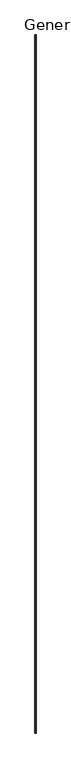
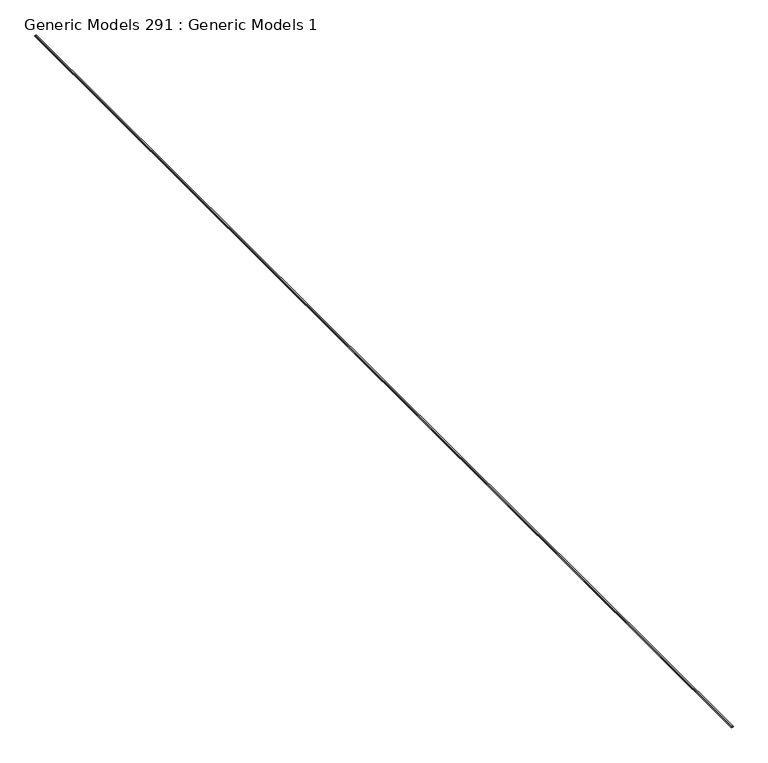
"""IFC4 building model written with IfcOpenShell, lengths in millimetres: proxy geometry, Generic Models 291 : Generic Models 1."""

import ifcopenshell
import ifcopenshell.guid

model = None  # the IFC model being written
_history = None  # IfcOwnerHistory: only IFC2X3 demands one
_inside = {}  # id of a spatial element -> (the spatial element, [elements in it])
_under = {}  # id of a project, library or spatial element -> (it, [spatial elements below it])
_declared = {}  # id of a project -> (the project, [libraries it declares])
_typed = {}  # id of a type object -> (the type object, [elements of that type])
_made_of = {}  # id of a material, layer set ... -> (it, [elements and type objects made of it])


def new_model(schema):
    """Start an empty IFC model of exactly this schema.

    Asked for "IFC4X3", IfcOpenShell would pick the latest addendum, in which some entities
    have other attributes; the version numbers below select the first issue.
    IFC2X3 requires an IfcOwnerHistory on every rooted entity: one is made here for all.
    """
    global model, _history
    if schema == "IFC4X3":
        model = ifcopenshell.file(schema_version=(4, 3, 0, 0))
    else:
        model = ifcopenshell.file(schema=schema)
    _inside.clear()
    _under.clear()
    _declared.clear()
    _typed.clear()
    _made_of.clear()
    _history = None
    if model.schema == "IFC2X3":
        org = make("IfcOrganization", Name="unknown")
        user = make(
            "IfcPersonAndOrganization",
            ThePerson=make("IfcPerson", FamilyName="unknown"),
            TheOrganization=org,
        )
        app = make(
            "IfcApplication",
            ApplicationDeveloper=org,
            Version="unknown",
            ApplicationFullName="unknown",
            ApplicationIdentifier="unknown",
        )
        _history = make(
            "IfcOwnerHistory",
            OwningUser=user,
            OwningApplication=app,
            ChangeAction="ADDED",
            CreationDate=0,
        )
    return model


def make(cls, **values):
    """One entity of the class cls with the attributes given. An attribute that is None is left unset."""
    return model.create_entity(
        cls, **{name: value for name, value in values.items() if value is not None}
    )


def rooted(cls, **values):
    """An entity with a GlobalId (a new one), such as an element, a storey or a relation."""
    return make(cls, GlobalId=ifcopenshell.guid.new(), OwnerHistory=_history, **values)


def si_unit(unit_type, name, prefix=None):
    """IfcSIUnit, for example si_unit("LENGTHUNIT", "METRE", prefix="MILLI")."""
    return make("IfcSIUnit", UnitType=unit_type, Prefix=prefix, Name=name)


def assignment(units):
    """IfcUnitAssignment: the units of a project."""
    return None if units is None else make("IfcUnitAssignment", Units=units)


def point(xyz):
    """IfcCartesianPoint."""
    return None if xyz is None else make("IfcCartesianPoint", Coordinates=xyz)


def direction(xyz):
    """IfcDirection."""
    return None if xyz is None else make("IfcDirection", DirectionRatios=xyz)


def frame(location, z_axis=None, x_axis=None):
    """IfcAxis2Placement3D, a coordinate frame: its origin and axes. An axis left out is left unset."""
    return make(
        "IfcAxis2Placement3D",
        Location=point(location),
        Axis=direction(z_axis),
        RefDirection=direction(x_axis),
    )


def origin():
    """The frame at (0, 0, 0) with its axes left unset."""
    return frame((0.0, 0.0, 0.0))


def place(relative_to, where):
    """IfcLocalPlacement: puts the frame where relative to a parent placement (None: the world)."""
    return make(
        "IfcLocalPlacement", PlacementRelTo=relative_to, RelativePlacement=where
    )


def context(
    kind, dimensions, precision=None, world=None, true_north=None, identifier=None
):
    """IfcGeometricRepresentationContext, for example the 3D "Model" context."""
    return make(
        "IfcGeometricRepresentationContext",
        ContextIdentifier=identifier,
        ContextType=kind,
        CoordinateSpaceDimension=dimensions,
        Precision=precision,
        WorldCoordinateSystem=world,
        TrueNorth=true_north,
    )


def project(units=None, contexts=None):
    """IfcProject with its units and contexts."""
    return rooted(
        "IfcProject",
        Name="project",
        RepresentationContexts=contexts,
        UnitsInContext=assignment(units),
    )


def spatial(cls, under=None, at=None, **own):
    """A site, building, storey or space (cls), placed at a placement, below another one or the project."""
    s = rooted(cls, ObjectPlacement=at, **own)
    if under is not None:
        _under.setdefault(under.id(), (under, []))[1].append(s)
    return s


def polyline(points):
    """IfcPolyline through the points."""
    return make("IfcPolyline", Points=[point(p) for p in points])


def circle_curve(where, radius):
    """IfcCircle in the frame where."""
    return make("IfcCircle", Position=where, Radius=radius)


def ellipse_curve(where, semi_axis1, semi_axis2):
    """IfcEllipse in the frame where."""
    return make(
        "IfcEllipse", Position=where, SemiAxis1=semi_axis1, SemiAxis2=semi_axis2
    )


def trimmed(basis, trim1, trim2, sense, master):
    """IfcTrimmedCurve: the piece of a basis curve between two trims."""
    return make(
        "IfcTrimmedCurve",
        BasisCurve=basis,
        Trim1=trim1,
        Trim2=trim2,
        SenseAgreement=sense,
        MasterRepresentation=master,
    )


def shape(context_of_items, identifier, shape_type, items):
    """IfcShapeRepresentation: the items that make up one representation, for example the "Body"."""
    return make(
        "IfcShapeRepresentation",
        ContextOfItems=context_of_items,
        RepresentationIdentifier=identifier,
        RepresentationType=shape_type,
        Items=items,
    )


def source(mapping_origin, context_of_items, identifier, shape_type, items):
    """IfcRepresentationMap: a shape defined once, which mapped items show again and again."""
    return make(
        "IfcRepresentationMap",
        MappingOrigin=mapping_origin,
        MappedRepresentation=shape(context_of_items, identifier, shape_type, items),
    )


def transform(
    local_origin,
    x_axis=None,
    y_axis=None,
    z_axis=None,
    scale=None,
    scale2=None,
    scale3=None,
    uniform=True,
):
    """IfcCartesianTransformationOperator3D, or its non-uniform kind. x_axis, y_axis, z_axis: its Axis1, 2, 3."""
    if uniform:
        return make(
            "IfcCartesianTransformationOperator3D",
            Axis1=direction(x_axis),
            Axis2=direction(y_axis),
            LocalOrigin=point(local_origin),
            Scale=scale,
            Axis3=direction(z_axis),
        )
    return make(
        "IfcCartesianTransformationOperator3DnonUniform",
        Axis1=direction(x_axis),
        Axis2=direction(y_axis),
        LocalOrigin=point(local_origin),
        Scale=scale,
        Axis3=direction(z_axis),
        Scale2=scale2,
        Scale3=scale3,
    )


def mapped(mapping_source, mapping_target):
    """IfcMappedItem: shows the shape of a source again, moved by a transform."""
    return make(
        "IfcMappedItem", MappingSource=mapping_source, MappingTarget=mapping_target
    )


def made_of(thing, what):
    """Note that an element or type object is made of a material, layer set ...; save() writes the relation."""
    if what is not None:
        _made_of.setdefault(what.id(), (what, []))[1].append(thing)
    return thing


def element(
    cls,
    number,
    at=None,
    inside=None,
    cuts=None,
    type_object=None,
    material=None,
    context=None,
    identifier="Body",
    shape_type=None,
    held_by="IfcProductDefinitionShape",
    body=None,
    shapes=None,
    **own,
):
    """One element of the class cls, such as IfcWall. Its Tag is "e" and its number.

    at: its placement. inside: the storey or other place that contains it. cuts: it is an
    opening in that element (IfcRelVoidsElement). A single representation is given by context,
    identifier, shape_type and body (its items); several are given by shapes. held_by: the class
    of the entity that holds the representations. save() writes the other relations.
    """
    e = rooted(cls, Tag="e%d" % number, ObjectPlacement=at, **own)
    if body is not None:
        shapes = [shape(context, identifier, shape_type, body)]
    if shapes is not None:
        e.Representation = make(held_by, Representations=shapes)
    if inside is not None:
        _inside.setdefault(inside.id(), (inside, []))[1].append(e)
    if cuts is not None:
        rooted(
            "IfcRelVoidsElement", RelatingBuildingElement=cuts, RelatedOpeningElement=e
        )
    if type_object is not None:
        _typed.setdefault(type_object.id(), (type_object, []))[1].append(e)
    return made_of(e, material)


def aggregate(whole, parts):
    """IfcRelAggregates: a whole, such as a stair, and the parts it consists of."""
    return rooted("IfcRelAggregates", RelatingObject=whole, RelatedObjects=parts)


def save(model, path):
    """Write the relations noted so far, then the file.

    IfcRelAggregates (storeys below a building ...), IfcRelContainedInSpatialStructure (elements
    in a storey), IfcRelDefinesByType, IfcRelAssociatesMaterial and IfcRelDeclares: one each for
    every whole, place, type object, material and project.
    """
    for whole, parts in _under.values():
        aggregate(whole, parts)
    for where, things in _inside.values():
        rooted(
            "IfcRelContainedInSpatialStructure",
            RelatedElements=things,
            RelatingStructure=where,
        )
    for kind, things in _typed.values():
        rooted("IfcRelDefinesByType", RelatedObjects=things, RelatingType=kind)
    for what, things in _made_of.values():
        rooted("IfcRelAssociatesMaterial", RelatedObjects=things, RelatingMaterial=what)
    for by, libraries in _declared.values():
        rooted("IfcRelDeclares", RelatingContext=by, RelatedDefinitions=libraries)
    model.write(path)


def plane_surface(at):
    """IfcPlane: the flat surface through the origin of the frame at, square to its z axis."""
    return make("IfcPlane", Position=at)


def cylinder_surface(at, radius):
    """IfcCylindricalSurface: all points at the distance radius from the z axis of the frame at."""
    return make("IfcCylindricalSurface", Position=at, Radius=radius)


def revolved_surface(curve, axis_point, axis_direction):
    """IfcSurfaceOfRevolution: the curve turned about the line through axis_point along axis_direction."""
    return make(
        "IfcSurfaceOfRevolution",
        SweptCurve=make("IfcArbitraryOpenProfileDef", ProfileType="CURVE", Curve=curve),
        AxisPosition=make("IfcAxis1Placement", Location=point(axis_point), Axis=direction(axis_direction)),
    )


def extruded_surface(curve, direction_of_extrusion, depth):
    """IfcSurfaceOfLinearExtrusion: the curve pushed along a direction by depth."""
    return make(
        "IfcSurfaceOfLinearExtrusion",
        SweptCurve=make("IfcArbitraryOpenProfileDef", ProfileType="CURVE", Curve=curve),
        ExtrudedDirection=direction(direction_of_extrusion),
        Depth=depth,
    )


def advanced_brep(points, edges, surfaces, faces):
    """IfcAdvancedBrep: a solid bounded by faces that lie on surfaces and meet in shared edges.

    An edge is (start, end): straight between two places in points (the first is 0);
    or (start, end, curve); or (start, end, curve, False) where it runs against its curve.
    A face is (place in surfaces, loops), or (place, loops, False) where it looks against
    its surface's normal. A loop lists edges by number (the first is 1), with a minus sign
    where the edge is run from its end to its start. The first loop is the outer one.
    """
    corners = [point(p) for p in points]
    vertices = [make("IfcVertexPoint", VertexGeometry=c) for c in corners]
    made = []
    for start, end, *more in edges:
        made.append(
            make(
                "IfcEdgeCurve",
                EdgeStart=vertices[start],
                EdgeEnd=vertices[end],
                EdgeGeometry=more[0] if more else make("IfcPolyline", Points=[corners[start], corners[end]]),
                SameSense=more[1] if len(more) > 1 else True,
            )
        )
    hull = []
    for where, loops, *sense in faces:
        bounds = []
        for j, loop in enumerate(loops):
            ring = [make("IfcOrientedEdge", EdgeElement=made[abs(k) - 1], Orientation=k > 0) for k in loop]
            bounds.append(
                make(
                    "IfcFaceOuterBound" if j == 0 else "IfcFaceBound",
                    Bound=make("IfcEdgeLoop", EdgeList=ring),
                    Orientation=True,
                )
            )
        hull.append(make("IfcAdvancedFace", Bounds=bounds, FaceSurface=surfaces[where], SameSense=sense[0] if sense else True))
    return make("IfcAdvancedBrep", Outer=make("IfcClosedShell", CfsFaces=hull))


def generic_models_291_generic_models_1_87a4b363(model_context):
    return source(origin(), model_context, "Body", "AdvancedBrep", [
        advanced_brep(
        [(4779.2187591, -1504.2676118, 129170.1348752), (4779.2187591, -1504.2676118, 129163.7848752), (4782.3937591, -1504.2676118, 129163.7848752), (4783.3455184, -1504.2676118, 129165.0555337), (4783.3455184, -1504.2676118, 129168.8642166), (4782.3937591, -1504.2676118, 129170.1348752), (4779.2187591, 6382.4323882, 129170.1348752), (4782.3937591, 6382.4323882, 129170.1348752), (4783.3455184, 6382.4323882, 129168.8642166), (4783.3455184, 6382.4323882, 129165.0555337), (4782.3937591, 6382.4323882, 129163.7848752), (4779.2187591, 6382.4323882, 129163.7848752)],
        [
            (0, 1, circle_curve(frame((4776.3040186, -1504.2676118, 129166.9598752), z_axis=(0.0, 1.0, 0.0), x_axis=(0.0, 0.0, 1.0)), 4.3100275)),
            (1, 2),
            (2, 3, circle_curve(frame((4779.4790186, -1504.2676118, 129166.9598752), z_axis=(0.0, -1.0, 0.0), x_axis=(0.0, 0.0, 1.0)), 4.3100275)),
            (3, 4, ellipse_curve(frame((4787.1562591, -1504.2676118, 129166.9598752), z_axis=(0.0, -1.0, 0.0), x_axis=(-1.0, 0.0, 0.0)), 4.7625, 3.175)),
            (4, 5, circle_curve(frame((4779.4790186, -1504.2676118, 129166.9598752), z_axis=(0.0, -1.0, 0.0), x_axis=(0.0, 0.0, 1.0)), 4.3100275)),
            (5, 0),
            (6, 7),
            (7, 8, circle_curve(frame((4779.4790186, 6382.4323882, 129166.9598752), z_axis=(0.0, 1.0, 0.0), x_axis=(0.0, 0.0, 1.0)), 4.3100275)),
            (8, 9, ellipse_curve(frame((4787.1562591, 6382.4323882, 129166.9598752), z_axis=(0.0, 1.0, 0.0), x_axis=(-1.0, 0.0, 0.0)), 4.7625, 3.175)),
            (9, 10, circle_curve(frame((4779.4790186, 6382.4323882, 129166.9598752), z_axis=(0.0, 1.0, 0.0), x_axis=(0.0, 0.0, 1.0)), 4.3100275)),
            (10, 11),
            (11, 6, circle_curve(frame((4776.3040186, 6382.4323882, 129166.9598752), z_axis=(0.0, -1.0, 0.0), x_axis=(0.0, 0.0, 1.0)), 4.3100275)),
            (3, 9),
            (8, 4),
            (5, 7),
            (6, 0),
            (2, 10),
            (1, 11),
        ],
        [
            plane_surface(frame((4779.2187591, -1504.2676118, 129163.7848752), z_axis=(0.0, -1.0, 0.0), x_axis=(-1.0, 0.0, 0.0))),
            plane_surface(frame((4779.2187591, 6382.4323882, 129163.7848752), z_axis=(0.0, 1.0, 0.0), x_axis=(-1.0, 0.0, 0.0))),
            extruded_surface(trimmed(ellipse_curve(frame((4787.1562591, 6382.4323882, 129166.9598752), z_axis=(0.0, -1.0, 0.0), x_axis=(-1.0, 0.0, 0.0)), 4.7625, 3.175), [point((4783.3455184, 6382.4323882, 129165.0555337))], [point((4783.3455184, 6382.4323882, 129168.8642166))], True, "CARTESIAN"), (0.0, -7886.7, 0.0), 7886.7),
            plane_surface(frame((4782.3937591, -1504.2676118, 129170.1348752), z_axis=(0.0, 0.0, 1.0), x_axis=(0.0, 1.0, 0.0))),
            cylinder_surface(frame((4779.4790186, -1504.2676118, 129166.9598752), z_axis=(0.0, -1.0, 0.0), x_axis=(0.0, 0.0, 1.0)), 4.3100275),
            plane_surface(frame((4779.2187591, -1504.2676118, 129163.7848752), z_axis=(0.0, 0.0, -1.0), x_axis=(0.0, 1.0, 0.0))),
            revolved_surface(polyline([(4776.3040186, 6382.4323882, 129171.2699027), (4776.3040186, -1504.2676118, 129171.2699027)]), (4776.3040186, -1504.2676118, 129166.9598752), (0.0, 1.0, 0.0)),
        ],
        [
            (0, [[1, 2, 3, 4, 5, 6]]),
            (1, [[7, 8, 9, 10, 11, 12]]),
            (2, [[-4, 13, -9, 14]]),
            (3, [[-6, 15, -7, 16]]),
            (4, [[-3, 17, -10, -13]]),
            (5, [[-2, 18, -11, -17]]),
            (6, [[-1, -16, -12, -18]]),
            (4, [[-5, -14, -8, -15]]),
        ],
    ),
    ])


if __name__ == "__main__":
    model = new_model("IFC4")
    model_context = context("Model", 3, world=origin())
    ifc_project = project(units=[si_unit("LENGTHUNIT", "METRE", prefix="MILLI")], contexts=[model_context])
    site = spatial("IfcSite", under=ifc_project)
    building = spatial("IfcBuilding", under=site)
    placement = place(None, origin())
    generic_models_291_generic_models_1_shape = generic_models_291_generic_models_1_87a4b363(model_context)
    element("IfcBuildingElementProxy", 1, Name="Generic Models 291 : Generic Models 1", ObjectType="Generic Models 291 : Generic Models 1", at=placement, inside=building, context=model_context, shape_type="MappedRepresentation", body=[
        mapped(generic_models_291_generic_models_1_shape, transform((0.0, 0.0, 0.0), x_axis=(1.0, 0.0, 0.0), y_axis=(0.0, 1.0, 0.0), z_axis=(0.0, 0.0, 1.0))),
    ])
    save(model, "model.ifc")

# Revit data of these elements
# Element 1 (IfcBuildingElementProxy, "Generic Models 291 : Generic Models 1")
#   Materials on its faces: "_SEALANT AND BACKROD, IF NEC."
# Materials
#   "_SEALANT AND BACKROD, IF NEC.": class "Generic", colour RGB 190 220 196, transparency 0, Cost = 0
